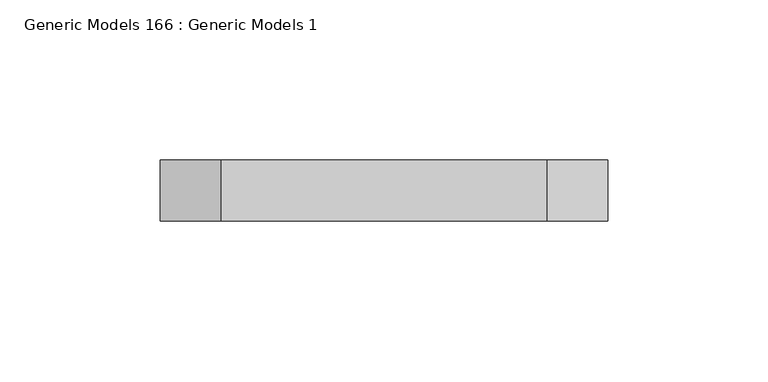
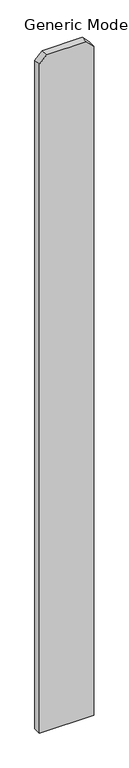
"""IFC4 building model written with IfcOpenShell, lengths in millimetres: proxy geometry, Generic Models 166 : Generic Models 1."""

from ifc_helpers import new_model, si_unit, frame, origin, place, context, project, spatial, polyline, outline, extrude, source, transform, mapped, element, save


def generic_models_166_generic_models_1_b867dca9(model_context):
    return source(origin(), model_context, "Body", "SweptSolid", [
        extrude(outline(polyline([(76.2, -249505.7875), (1885.95, -249505.7875), (1905.0, -249524.8375), (1905.0, -249626.4375), (1885.95, -249645.4875), (76.2, -249645.4875), (76.2, -249505.7875)])), frame((0.0, 547.6875, 0.0), z_axis=(0.0, 1.0, 0.0), x_axis=(0.0, 0.0, 1.0)), (0.0, 0.0, 1.0), 19.05),
    ])


if __name__ == "__main__":
    model = new_model("IFC4")
    model_context = context("Model", 3, world=origin())
    ifc_project = project(units=[si_unit("LENGTHUNIT", "METRE", prefix="MILLI")], contexts=[model_context])
    site = spatial("IfcSite", under=ifc_project)
    building = spatial("IfcBuilding", under=site)
    placement = place(None, origin())
    generic_models_166_generic_models_1_shape = generic_models_166_generic_models_1_b867dca9(model_context)
    element("IfcBuildingElementProxy", 1, Name="Generic Models 166 : Generic Models 1", ObjectType="Generic Models 166 : Generic Models 1", at=placement, inside=building, context=model_context, shape_type="MappedRepresentation", body=[
        mapped(generic_models_166_generic_models_1_shape, transform((0.0, 0.0, 0.0), x_axis=(1.0, 0.0, 0.0), y_axis=(0.0, 1.0, 0.0), z_axis=(0.0, 0.0, 1.0))),
    ])
    save(model, "model.ifc")

# Revit data of these elements
# Element 1 (IfcBuildingElementProxy, "Generic Models 166 : Generic Models 1")
#   Materials on its faces: "VERTICAL 1X6 CEDAR PLANKS W/ CLEAR WOOD SEALER"
# Materials
#   "VERTICAL 1X6 CEDAR PLANKS W/ CLEAR WOOD SEALER": class "Wood", colour RGB 234 198 147, transparency 0, Description = "Pinus Echinata", Cost = 0
